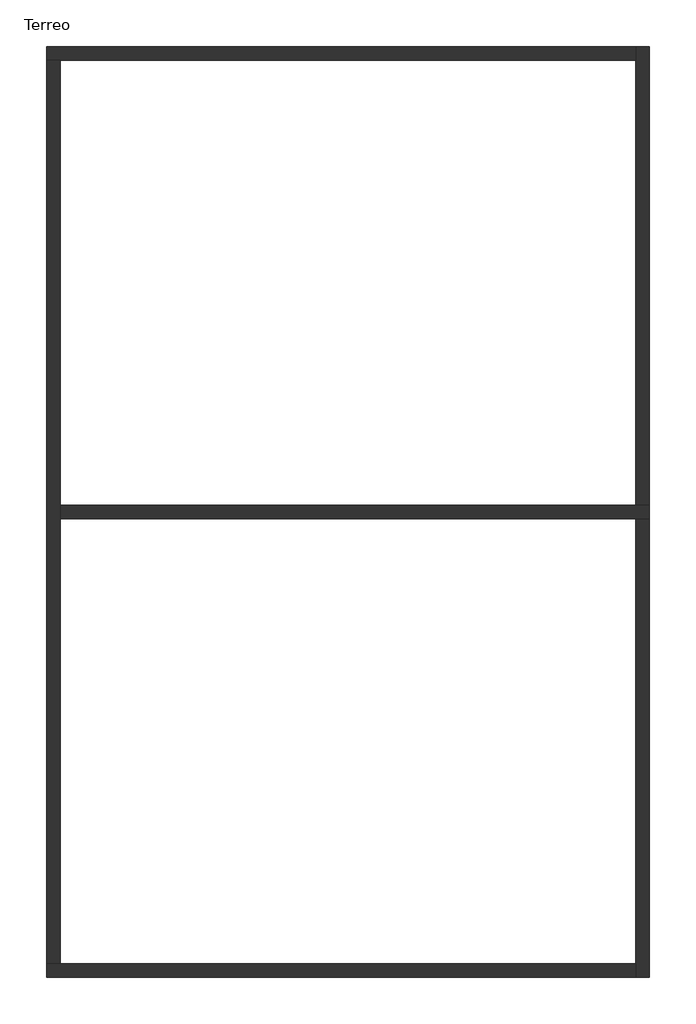
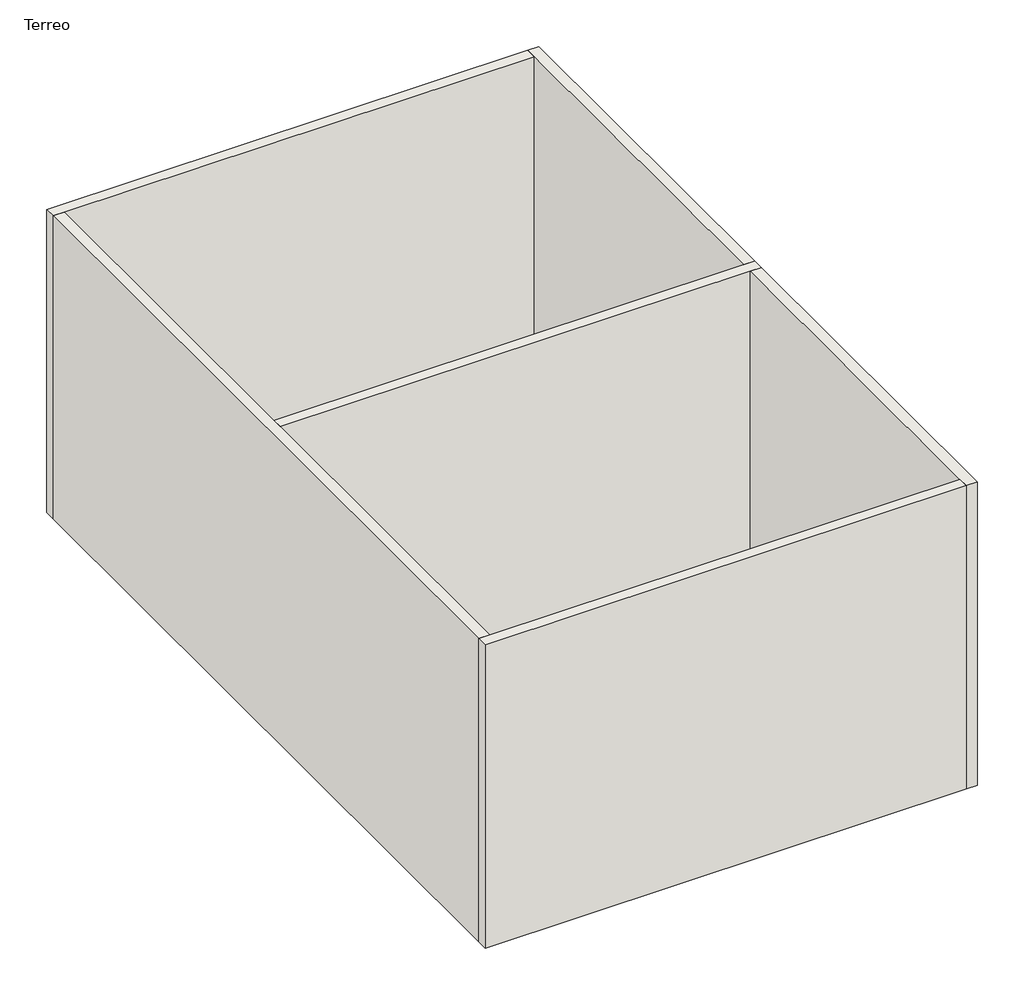
# One storey: 7 walls.
"""IFC4 building model written with IfcOpenShell, lengths in millimetres."""

import ifcopenshell
import ifcopenshell.guid

model = None  # the IFC model being written
_history = None  # IfcOwnerHistory: only IFC2X3 demands one
_inside = {}  # id of a spatial element -> (the spatial element, [elements in it])
_under = {}  # id of a project, library or spatial element -> (it, [spatial elements below it])
_declared = {}  # id of a project -> (the project, [libraries it declares])
_typed = {}  # id of a type object -> (the type object, [elements of that type])
_made_of = {}  # id of a material, layer set ... -> (it, [elements and type objects made of it])


def new_model(schema):
    """Start an empty IFC model of exactly this schema.

    Asked for "IFC4X3", IfcOpenShell would pick the latest addendum, in which some entities
    have other attributes; the version numbers below select the first issue.
    IFC2X3 requires an IfcOwnerHistory on every rooted entity: one is made here for all.
    """
    global model, _history
    if schema == "IFC4X3":
        model = ifcopenshell.file(schema_version=(4, 3, 0, 0))
    else:
        model = ifcopenshell.file(schema=schema)
    _inside.clear()
    _under.clear()
    _declared.clear()
    _typed.clear()
    _made_of.clear()
    _history = None
    if model.schema == "IFC2X3":
        org = make("IfcOrganization", Name="unknown")
        user = make(
            "IfcPersonAndOrganization",
            ThePerson=make("IfcPerson", FamilyName="unknown"),
            TheOrganization=org,
        )
        app = make(
            "IfcApplication",
            ApplicationDeveloper=org,
            Version="unknown",
            ApplicationFullName="unknown",
            ApplicationIdentifier="unknown",
        )
        _history = make(
            "IfcOwnerHistory",
            OwningUser=user,
            OwningApplication=app,
            ChangeAction="ADDED",
            CreationDate=0,
        )
    return model


def make(cls, **values):
    """One entity of the class cls with the attributes given. An attribute that is None is left unset."""
    return model.create_entity(
        cls, **{name: value for name, value in values.items() if value is not None}
    )


def rooted(cls, **values):
    """An entity with a GlobalId (a new one), such as an element, a storey or a relation."""
    return make(cls, GlobalId=ifcopenshell.guid.new(), OwnerHistory=_history, **values)


def si_unit(unit_type, name, prefix=None):
    """IfcSIUnit, for example si_unit("LENGTHUNIT", "METRE", prefix="MILLI")."""
    return make("IfcSIUnit", UnitType=unit_type, Prefix=prefix, Name=name)


def assignment(units):
    """IfcUnitAssignment: the units of a project."""
    return None if units is None else make("IfcUnitAssignment", Units=units)


def point(xyz):
    """IfcCartesianPoint."""
    return None if xyz is None else make("IfcCartesianPoint", Coordinates=xyz)


def direction(xyz):
    """IfcDirection."""
    return None if xyz is None else make("IfcDirection", DirectionRatios=xyz)


def frame(location, z_axis=None, x_axis=None):
    """IfcAxis2Placement3D, a coordinate frame: its origin and axes. An axis left out is left unset."""
    return make(
        "IfcAxis2Placement3D",
        Location=point(location),
        Axis=direction(z_axis),
        RefDirection=direction(x_axis),
    )


def origin():
    """The frame at (0, 0, 0) with its axes left unset."""
    return frame((0.0, 0.0, 0.0))


def place(relative_to, where):
    """IfcLocalPlacement: puts the frame where relative to a parent placement (None: the world)."""
    return make(
        "IfcLocalPlacement", PlacementRelTo=relative_to, RelativePlacement=where
    )


def context(
    kind, dimensions, precision=None, world=None, true_north=None, identifier=None
):
    """IfcGeometricRepresentationContext, for example the 3D "Model" context."""
    return make(
        "IfcGeometricRepresentationContext",
        ContextIdentifier=identifier,
        ContextType=kind,
        CoordinateSpaceDimension=dimensions,
        Precision=precision,
        WorldCoordinateSystem=world,
        TrueNorth=true_north,
    )


def project(units=None, contexts=None):
    """IfcProject with its units and contexts."""
    return rooted(
        "IfcProject",
        Name="project",
        RepresentationContexts=contexts,
        UnitsInContext=assignment(units),
    )


def spatial(cls, under=None, at=None, **own):
    """A site, building, storey or space (cls), placed at a placement, below another one or the project."""
    s = rooted(cls, ObjectPlacement=at, **own)
    if under is not None:
        _under.setdefault(under.id(), (under, []))[1].append(s)
    return s


def faces_of(points, faces, orient=None, outer=None):
    """IfcFace entities. A face is a list of loops; a loop is a list of indices into points, from 0.

    orient and outer hold one flag for each loop. By default every Orientation is true, the
    first loop of a face is its IfcFaceOuterBound and the others are IfcFaceBound.
    """
    made = []
    for i, loops in enumerate(faces):
        bounds = []
        for j, loop in enumerate(loops):
            is_outer = j == 0 if outer is None else outer[i][j]
            bounds.append(
                make(
                    "IfcFaceOuterBound" if is_outer else "IfcFaceBound",
                    Bound=make("IfcPolyLoop", Polygon=[points[k] for k in loop]),
                    Orientation=True if orient is None else orient[i][j],
                )
            )
        made.append(make("IfcFace", Bounds=bounds))
    return made


def faceted_brep(points, faces, orient=None, outer=None, voids=None):
    """IfcFacetedBrep: a solid bounded by flat faces; with voids (closed shells), ...WithVoids."""
    shared = [point(p) for p in points]
    hull = make("IfcClosedShell", CfsFaces=faces_of(shared, faces, orient, outer))
    if voids is None:
        return make("IfcFacetedBrep", Outer=hull)
    return make(
        "IfcFacetedBrepWithVoids",
        Outer=hull,
        Voids=[
            make(cls, CfsFaces=faces_of(shared, fs, o, b)) for cls, fs, o, b in voids
        ],
    )


def shape(context_of_items, identifier, shape_type, items):
    """IfcShapeRepresentation: the items that make up one representation, for example the "Body"."""
    return make(
        "IfcShapeRepresentation",
        ContextOfItems=context_of_items,
        RepresentationIdentifier=identifier,
        RepresentationType=shape_type,
        Items=items,
    )


def made_of(thing, what):
    """Note that an element or type object is made of a material, layer set ...; save() writes the relation."""
    if what is not None:
        _made_of.setdefault(what.id(), (what, []))[1].append(thing)
    return thing


def element(
    cls,
    number,
    at=None,
    inside=None,
    cuts=None,
    type_object=None,
    material=None,
    context=None,
    identifier="Body",
    shape_type=None,
    held_by="IfcProductDefinitionShape",
    body=None,
    shapes=None,
    **own,
):
    """One element of the class cls, such as IfcWall. Its Tag is "e" and its number.

    at: its placement. inside: the storey or other place that contains it. cuts: it is an
    opening in that element (IfcRelVoidsElement). A single representation is given by context,
    identifier, shape_type and body (its items); several are given by shapes. held_by: the class
    of the entity that holds the representations. save() writes the other relations.
    """
    e = rooted(cls, Tag="e%d" % number, ObjectPlacement=at, **own)
    if body is not None:
        shapes = [shape(context, identifier, shape_type, body)]
    if shapes is not None:
        e.Representation = make(held_by, Representations=shapes)
    if inside is not None:
        _inside.setdefault(inside.id(), (inside, []))[1].append(e)
    if cuts is not None:
        rooted(
            "IfcRelVoidsElement", RelatingBuildingElement=cuts, RelatedOpeningElement=e
        )
    if type_object is not None:
        _typed.setdefault(type_object.id(), (type_object, []))[1].append(e)
    return made_of(e, material)


def aggregate(whole, parts):
    """IfcRelAggregates: a whole, such as a stair, and the parts it consists of."""
    return rooted("IfcRelAggregates", RelatingObject=whole, RelatedObjects=parts)


def save(model, path):
    """Write the relations noted so far, then the file.

    IfcRelAggregates (storeys below a building ...), IfcRelContainedInSpatialStructure (elements
    in a storey), IfcRelDefinesByType, IfcRelAssociatesMaterial and IfcRelDeclares: one each for
    every whole, place, type object, material and project.
    """
    for whole, parts in _under.values():
        aggregate(whole, parts)
    for where, things in _inside.values():
        rooted(
            "IfcRelContainedInSpatialStructure",
            RelatedElements=things,
            RelatingStructure=where,
        )
    for kind, things in _typed.values():
        rooted("IfcRelDefinesByType", RelatedObjects=things, RelatingType=kind)
    for what, things in _made_of.values():
        rooted("IfcRelAssociatesMaterial", RelatedObjects=things, RelatingMaterial=what)
    for by, libraries in _declared.values():
        rooted("IfcRelDeclares", RelatingContext=by, RelatedDefinitions=libraries)
    model.write(path)


model = new_model("IFC4")

# Units and contexts
model_context = context("Model", 3, world=origin())
ifc_project = project(units=[si_unit("LENGTHUNIT", "METRE", prefix="MILLI")], contexts=[model_context])

# Site, building, storey
site = spatial("IfcSite", under=ifc_project)
building = spatial("IfcBuilding", under=site)
storey = spatial("IfcBuildingStorey", under=building, Name="Terreo", Elevation=0.0)

# Walls
placement = place(None, origin())
element("IfcWall", 1, ObjectType="Parede 19 cm - Pintura / Pintura", at=placement, inside=storey, context=model_context, shape_type="Brep", body=[
    faceted_brep([(-5341.8408024, 6777.0494336, 0.0), (3448.9591976, 6777.0494336, 0.0), (3658.1591976, 6777.0494336, 0.0), (3658.1591976, 6777.0494336, 6000.0), (3448.9591976, 6777.0494336, 6000.0), (-5341.8408024, 6777.0494336, 6000.0), (-5341.8408024, 6986.2494336, 0.0), (-5341.8408024, 6986.2494336, 6000.0), (3448.9591976, 6986.2494336, 6000.0), (3658.1591976, 6986.2494336, 6000.0), (3658.1591976, 6986.2494336, 0.0), (3448.9591976, 6986.2494336, 0.0)], [[[0, 1, 2, 3, 4, 5]], [[6, 7, 8, 9, 10, 11]], [[2, 1, 0, 6, 11, 10]], [[5, 4, 3, 9, 8, 7]], [[3, 2, 10, 9]], [[0, 5, 7, 6]]]),
])
element("IfcWall", 2, ObjectType="Parede 19 cm - Pintura / Pintura", at=placement, inside=storey, context=model_context, shape_type="Brep", body=[
    faceted_brep([(3448.9591976, 6777.0494336, 0.0), (3448.9591976, -13.7505664, 0.0), (3448.9591976, -222.9505664, 0.0), (3448.9591976, -222.9505664, 6000.0), (3448.9591976, -13.7505664, 6000.0), (3448.9591976, 6777.0494336, 6000.0), (3658.1591976, 6777.0494336, 0.0), (3658.1591976, 6777.0494336, 6000.0), (3658.1591976, -222.9505664, 6000.0), (3658.1591976, -222.9505664, 0.0)], [[[0, 1, 2, 3, 4, 5]], [[6, 7, 8, 9]], [[2, 1, 0, 6, 9]], [[5, 4, 3, 8, 7]], [[0, 5, 7, 6]], [[3, 2, 9, 8]]]),
])
element("IfcWall", 3, ObjectType="Parede 19 cm - Pintura / Pintura", at=placement, inside=storey, context=model_context, shape_type="Brep", body=[
    faceted_brep([(3448.9591976, -13.7505664, 0.0), (-5341.8408024, -13.7505664, 0.0), (-5551.0408024, -13.7505664, 0.0), (-5551.0408024, -13.7505664, 6000.0), (-5341.8408024, -13.7505664, 6000.0), (3448.9591976, -13.7505664, 6000.0), (3448.9591976, -222.9505664, 0.0), (3448.9591976, -222.9505664, 6000.0), (-5551.0408024, -222.9505664, 6000.0), (-5551.0408024, -222.9505664, 0.0)], [[[0, 1, 2, 3, 4, 5]], [[6, 7, 8, 9]], [[2, 1, 0, 6, 9]], [[5, 4, 3, 8, 7]], [[0, 5, 7, 6]], [[3, 2, 9, 8]]]),
])
element("IfcWall", 4, ObjectType="Parede 19 cm - Pintura / Pintura", at=placement, inside=storey, context=model_context, shape_type="Brep", body=[
    faceted_brep([(-5341.8408024, -13.7505664, 0.0), (-5341.8408024, 6777.0494336, 0.0), (-5341.8408024, 6986.2494336, 0.0), (-5341.8408024, 13777.0494336, 0.0), (-5341.8408024, 13777.0494336, 6000.0), (-5341.8408024, 6986.2494336, 6000.0), (-5341.8408024, 6777.0494336, 6000.0), (-5341.8408024, -13.7505664, 6000.0), (-5551.0408024, -13.7505664, 0.0), (-5551.0408024, -13.7505664, 6000.0), (-5551.0408024, 13777.0494336, 6000.0), (-5551.0408024, 13777.0494336, 0.0)], [[[0, 1, 2, 3, 4, 5, 6, 7]], [[8, 9, 10, 11]], [[3, 2, 1, 0, 8, 11]], [[7, 6, 5, 4, 10, 9]], [[0, 7, 9, 8]], [[4, 3, 11, 10]]]),
])
element("IfcWall", 5, ObjectType="Parede 19 cm - Pintura / Pintura", at=placement, inside=storey, context=model_context, shape_type="Brep", body=[
    faceted_brep([(3658.1591976, 6986.2494336, 0.0), (3658.1591976, 13986.2494336, 0.0), (3658.1591976, 13986.2494336, 6000.0), (3658.1591976, 6986.2494336, 6000.0), (3448.9591976, 6986.2494336, 0.0), (3448.9591976, 6986.2494336, 6000.0), (3448.9591976, 13777.0494336, 6000.0), (3448.9591976, 13986.2494336, 6000.0), (3448.9591976, 13986.2494336, 0.0), (3448.9591976, 13777.0494336, 0.0)], [[[0, 1, 2, 3]], [[4, 5, 6, 7, 8, 9]], [[1, 0, 4, 9, 8]], [[3, 2, 7, 6, 5]], [[2, 1, 8, 7]], [[0, 3, 5, 4]]]),
])
element("IfcWall", 6, ObjectType="Parede 19 cm - Pintura / Pintura", at=placement, inside=storey, context=model_context, shape_type="Brep", body=[
    faceted_brep([(3448.9591976, 13986.2494336, 0.0), (-5551.0408024, 13986.2494336, 0.0), (-5551.0408024, 13986.2494336, 6000.0), (3448.9591976, 13986.2494336, 6000.0), (3448.9591976, 13777.0494336, 0.0), (3448.9591976, 13777.0494336, 6000.0), (-5341.8408024, 13777.0494336, 6000.0), (-5551.0408024, 13777.0494336, 6000.0), (-5551.0408024, 13777.0494336, 0.0), (-5341.8408024, 13777.0494336, 0.0)], [[[0, 1, 2, 3]], [[4, 5, 6, 7, 8, 9]], [[1, 0, 4, 9, 8]], [[3, 2, 7, 6, 5]], [[0, 3, 5, 4]], [[2, 1, 8, 7]]]),
])
element("IfcWall", 7, ObjectType="Parede 19 cm - Pintura / Pintura", at=placement, inside=storey, context=model_context, shape_type="Brep", body=[
    faceted_brep([(-5551.0408024, 13777.0494336, 0.0), (-5341.8408024, 13777.0494336, 0.0), (3448.9591976, 13777.0494336, 0.0), (3448.9591976, 13777.0494336, 6000.0), (-5341.8408024, 13777.0494336, 6000.0), (-5551.0408024, 13777.0494336, 6000.0), (-5551.0408024, 13986.2494336, 0.0), (-5551.0408024, 13986.2494336, 6000.0), (3448.9591976, 13986.2494336, 6000.0), (3448.9591976, 13986.2494336, 0.0)], [[[0, 1, 2, 3, 4, 5]], [[6, 7, 8, 9]], [[2, 1, 0, 6, 9]], [[5, 4, 3, 8, 7]], [[3, 2, 9, 8]], [[0, 5, 7, 6]]]),
])

save(model, "model.ifc")

# Revit data of these elements
# Project information
#   Project Issue Date = "Data de emissão"
#   Project Status = "Status do projeto"
#   Client Name = "Proprietário"
#   Project Address = "Insira aqui o endereço"
#   Project Name = "Nome do projeto"
#   Project Number = "0001"
# Type "Parede 19 cm - Pintura / Pintura"
#   Width = 0.2092 m
#   Layers, outside or top first: 0.0016 m "Pintura Látex PVA" (function 4); 0.008 m "Gesso" (function 4); 0.19 m "Alvenaria - Bloco de Cerâmico - 14cm" (function 1); 0.008 m "Gesso" (function 2); 0.0016 m "Pintura Látex PVA" (function 4)
# Elements 1, 2, 3, 5, 6, 7 (IfcWall, "Parede 19 cm - Pintura / Pintura")
#   Top Offset = 0.00 m
#   Base Offset = 0.00 m
#   wall height = 6.00 m
#   Phase Created = Construção nova
#   Base Constraint = Terreo
#   Top Constraint = Cobertura
#   Materials on its faces: "Pintura Látex PVA", "Material pré-definido de parede"
# Element 4 (IfcWall, "Parede 19 cm - Pintura / Pintura")
#   Top Offset = 0.00 m
#   Base Offset = 0.00 m
#   wall height = 6.00 m
#   Phase Created = Construção nova
#   Base Constraint = Terreo
#   Top Constraint = Cobertura
#   Materials on its faces: "Material pré-definido de parede", "Pintura Látex PVA"
# Materials
#   "Pintura Látex PVA": class "Pintura", colour RGB 244 244 244, transparency 0, Cost = 0
#   "Gesso": class "Gesso", colour RGB 244 244 244, transparency 0, Cost = 0
#   "Alvenaria - Bloco de Cerâmico - 14cm": class "Cerâmica", colour RGB 255 255 255, transparency 0, Cost = 0
#   "Material pré-definido de parede": class "Diversos", colour RGB 128 128 128, transparency 0
